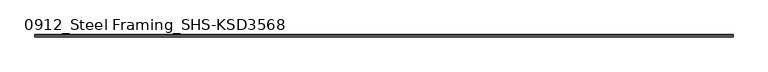
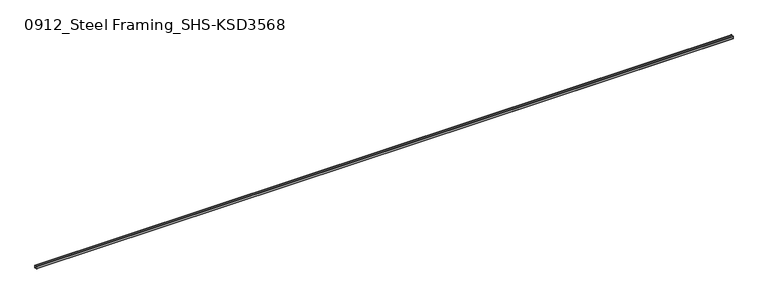
"""IFC4 building model written with IfcOpenShell, lengths in millimetres: beam geometry, 0912_Steel Framing_SHS-KSD3568 : H_SB_ASB_SHS-150x150x6."""

from ifc_helpers import new_model, si_unit, point, frame, frame_2d, origin, place, context, project, spatial, polyline, circle_curve, trimmed, segment, composite_curve, outline, extrude, source, transform, mapped, element, save


def beam_0912_steel_framing_shs_ksd3568_e6cc96f6(model_context):
    return source(origin(), model_context, "Body", "SweptSolid", [
        extrude(outline(composite_curve([segment(polyline([(75.0, 63.0), (75.0, -63.0)]), True, "CONTINUOUS"), segment(trimmed(circle_curve(frame_2d((63.0, -63.0)), 12.0), [point((75.0, -63.0))], [point((63.0, -75.0))], False, "CARTESIAN"), True, "CONTINUOUS"), segment(polyline([(63.0, -75.0), (-63.0, -75.0)]), True, "CONTINUOUS"), segment(trimmed(circle_curve(frame_2d((-63.0, -63.0)), 12.0), [point((-63.0, -75.0))], [point((-75.0, -63.0))], False, "CARTESIAN"), True, "CONTINUOUS"), segment(polyline([(-75.0, -63.0), (-75.0, 63.0)]), True, "CONTINUOUS"), segment(trimmed(circle_curve(frame_2d((-63.0, 63.0)), 12.0), [point((-75.0, 63.0))], [point((-63.0, 75.0))], False, "CARTESIAN"), True, "CONTINUOUS"), segment(polyline([(-63.0, 75.0), (63.0, 75.0)]), True, "CONTINUOUS"), segment(trimmed(circle_curve(frame_2d((63.0, 63.0)), 12.0), [point((63.0, 75.0))], [point((75.0, 63.0))], False, "CARTESIAN"), True, "CONTINUOUS")], self_intersect=False), holes=[composite_curve([segment(trimmed(circle_curve(frame_2d((-63.0, 63.0)), 6.0), [point((-63.0, 69.0))], [point((-69.0, 63.0))], True, "CARTESIAN"), True, "CONTINUOUS"), segment(polyline([(-69.0, 63.0), (-69.0, -63.0)]), True, "CONTINUOUS"), segment(trimmed(circle_curve(frame_2d((-63.0, -63.0)), 6.0), [point((-69.0, -63.0))], [point((-63.0, -69.0))], True, "CARTESIAN"), True, "CONTINUOUS"), segment(polyline([(-63.0, -69.0), (63.0, -69.0)]), True, "CONTINUOUS"), segment(trimmed(circle_curve(frame_2d((63.0, -63.0)), 6.0), [point((63.0, -69.0))], [point((69.0, -63.0))], True, "CARTESIAN"), True, "CONTINUOUS"), segment(polyline([(69.0, -63.0), (69.0, 63.0)]), True, "CONTINUOUS"), segment(trimmed(circle_curve(frame_2d((63.0, 63.0)), 6.0), [point((69.0, 63.0))], [point((63.0, 69.0))], True, "CARTESIAN"), True, "CONTINUOUS"), segment(polyline([(63.0, 69.0), (-63.0, 69.0)]), True, "CONTINUOUS")], self_intersect=False)]), frame((-20462.3, 0.0, 0.0), z_axis=(1.0, 0.0, 0.0), x_axis=(0.0, 1.0, 0.0)), (0.0, 0.0, 1.0), 40924.6),
    ])


if __name__ == "__main__":
    model = new_model("IFC4")
    model_context = context("Model", 3, world=origin())
    ifc_project = project(units=[si_unit("LENGTHUNIT", "METRE", prefix="MILLI")], contexts=[model_context])
    site = spatial("IfcSite", under=ifc_project)
    building = spatial("IfcBuilding", under=site)
    placement = place(None, origin())
    beam_0912_steel_framing_shs_ksd3568_shape = beam_0912_steel_framing_shs_ksd3568_e6cc96f6(model_context)
    element("IfcBeam", 1, ObjectType="0912_Steel Framing_SHS-KSD3568 : H_SB_ASB_SHS-150x150x6", at=placement, inside=building, context=model_context, shape_type="MappedRepresentation", body=[
        mapped(beam_0912_steel_framing_shs_ksd3568_shape, transform((0.0, 0.0, 0.0), x_axis=(1.0, 0.0, 0.0), y_axis=(0.0, 1.0, 0.0), z_axis=(0.0, 0.0, 1.0))),
    ])
    save(model, "model.ifc")

# Revit data of these elements
# Type "0912_Steel Framing_SHS-KSD3568 : H_SB_ASB_SHS-150x150x6"
#   H_WM Code_1 = "S01AA002-00001 | Main Steel Structure Fabrication Work | Shelter/Building | Medium Steel - Standard (90KG/M>Weight≥30KG/M) | Material: (   )"
#   H_WM Code_2 = "S03AA028-00001 | Main Steel Structure Erection Work | Shelter/Building | Medium Steel (90KG/M>Weight≥30KG/M) | Material: (   )"
#   H_WM Code_3 = "S01AA010-00001 | Main Steel Structure Fabrication Work | Shelter/Building | Steel Painting/Coating | for Non-Fireproofed Steel Surface, Surface Preparation, Primer, Second & Final Coat | Material: (   )"
#   H_Q'ty Cal Type Tag = "SB-Q2"
#   Perimeter = 0.60 m²/m
#   Nominal Weight = 26.40 kgf/m
#   Length [instance default] = 1.0000 m
#   b = 0.1500 m
#   h = 0.1500 m
#   tr = 0.0120 m
#   t = 0.0060 m
#   A = 28.36 m²
#   Structural Material [instance default] = Steel, 45-345
# Element 1 (IfcBeam, "0912_Steel Framing_SHS-KSD3568 : H_SB_ASB_SHS-150x150x6")
#   Structural Material = none
# Materials
#   "Steel, 45-345": class "Metal", colour RGB 189 187 185, transparency 0, Description = "Steel 345 MPa", Cost = 0
